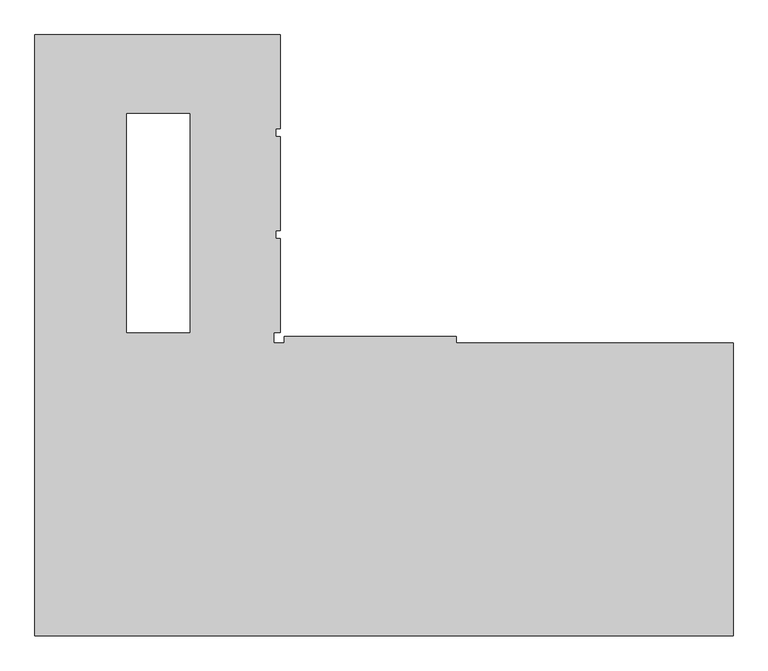
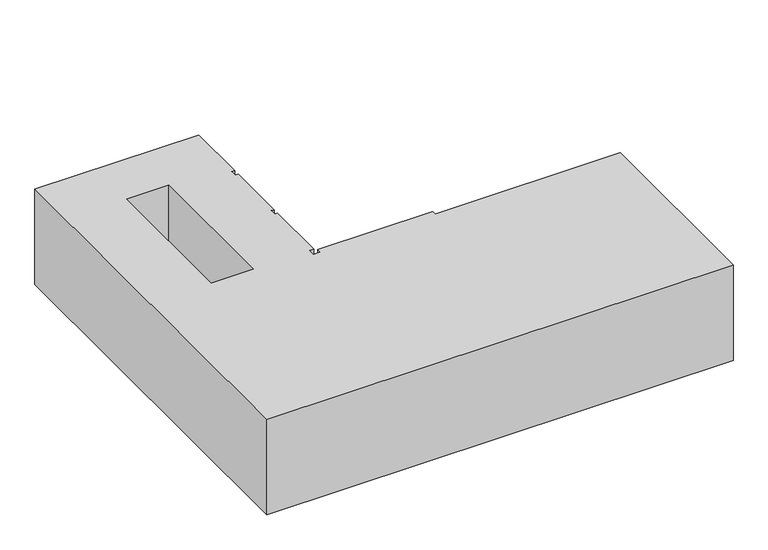
"""IFC4 building model written with IfcOpenShell, lengths in millimetres: proxy geometry, 0_3d_modell."""

from ifc_helpers import new_model, si_unit, origin, origin_with_axes, place, context, project, spatial, polyline, outline, extrude, source, transform, mapped, element, save


def generic_models_b5a4028e(model_context):
    return source(origin(), model_context, "Body", "SweptSolid", [
        extrude(outline(polyline([(4550.0, 5582.8619019), (4750.0, 5582.8619019), (4750.0, 5704.8619019), (8028.0, 5704.8619019), (8028.0, 5582.8619019), (13300.0, 5582.8619019), (13300.0, 0.0), (0.0, 0.0), (0.0, 11452.8619019), (4672.0, 11452.8619019), (4672.0, 9669.4619019), (4590.0, 9669.4619019), (4590.0, 9509.4619019), (4672.0, 9509.4619019), (4672.0, 7726.1619019), (4590.0, 7726.1619019), (4590.0, 7566.1619019), (4672.0, 7566.1619019), (4672.0, 5782.8619019), (4550.0, 5782.8619019), (4550.0, 5582.8619019)]), holes=[polyline([(2949.4613155, 5782.8619019), (2949.4613155, 9952.8619019), (1748.7090817, 9952.8619019), (1748.7090817, 5782.8619019), (2949.4613155, 5782.8619019)])]), origin_with_axes(), (0.0, 0.0, 1.0), 2880.0),
    ])


if __name__ == "__main__":
    model = new_model("IFC4")
    model_context = context("Model", 3, world=origin())
    ifc_project = project(units=[si_unit("LENGTHUNIT", "METRE", prefix="MILLI")], contexts=[model_context])
    site = spatial("IfcSite", under=ifc_project)
    building = spatial("IfcBuilding", under=site)
    placement = place(None, origin())
    generic_models_shape = generic_models_b5a4028e(model_context)
    element("IfcBuildingElementProxy", 1, Name="0_3d_modell", ObjectType="0_3d_modell", at=placement, inside=building, context=model_context, shape_type="MappedRepresentation", body=[
        mapped(generic_models_shape, transform((0.0, 0.0, 0.0), x_axis=(1.0, 0.0, 0.0), y_axis=(0.0, 1.0, 0.0), z_axis=(0.0, 0.0, 1.0))),
    ])
    save(model, "model.ifc")

# Revit data of these elements
# Element 1 (IfcBuildingElementProxy, "0_3d_modell")
#   Materials on its faces: "*1"
# Materials
#   "*1": class "Unassigned", colour RGB 175 175 175, transparency 0
